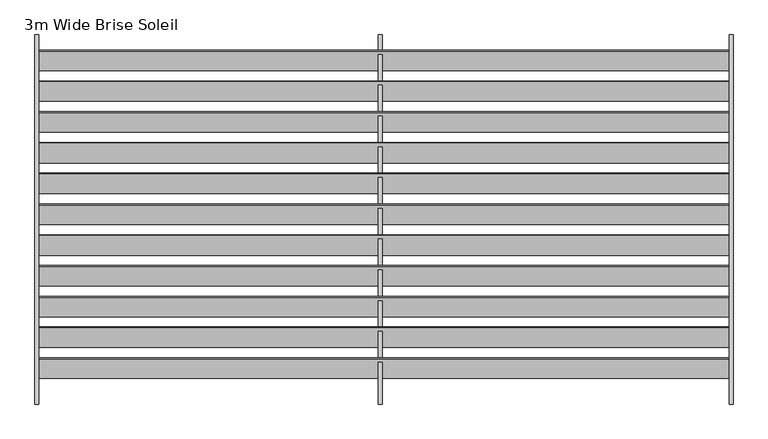
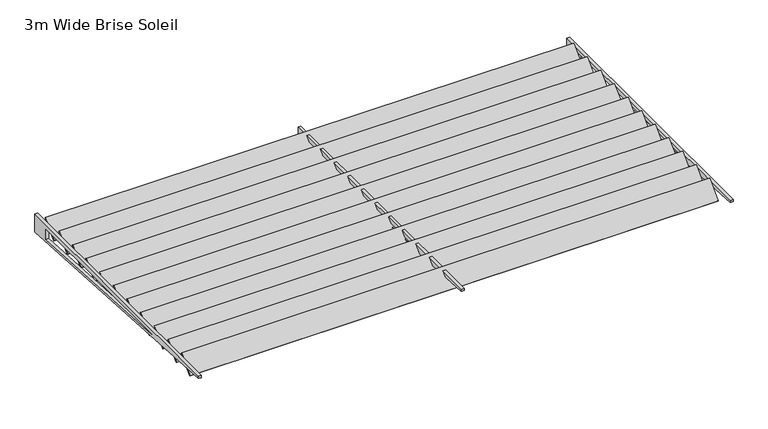
"""IFC4 building model written with IfcOpenShell, lengths in millimetres: railing geometry, 3m Wide Brise Soleil."""

from ifc_helpers import new_model, si_unit, frame, origin, place, context, project, spatial, polyline, outline, extrude, source, transform, mapped, element, save


def railing_3m_wide_brise_soleil_33fbfd34(model_context):
    return source(origin(), model_context, "Body", "SweptSolid", [
        extrude(outline(polyline([(0.0, -10.0), (0.0, 0.0), (5596.1382149, 0.0), (5596.1382149, -10.0), (0.0, -10.0)])), frame((4426.8341559, -31953.9338219, -139.965894), z_axis=(0.0, 0.7071067811931987, 0.7071067811798963), x_axis=(1.0, 0.0, 0.0)), (0.0, 0.0, 1.0), 225.0),
        extrude(outline(polyline([(0.0, -10.0), (0.0, 0.0), (5596.1382149, 0.0), (5596.1382149, -10.0), (0.0, -10.0)])), frame((4426.8341559, -31703.9338219, -139.965894), z_axis=(0.0, 0.7071067811931987, 0.7071067811798963), x_axis=(1.0, 0.0, 0.0)), (0.0, 0.0, 1.0), 225.0),
        extrude(outline(polyline([(0.0, -10.0), (0.0, 0.0), (5596.1382149, 0.0), (5596.1382149, -10.0), (0.0, -10.0)])), frame((4426.8341559, -31453.9338219, -139.965894), z_axis=(0.0, 0.7071067811931987, 0.7071067811798963), x_axis=(1.0, 0.0, 0.0)), (0.0, 0.0, 1.0), 225.0),
        extrude(outline(polyline([(0.0, -10.0), (0.0, 0.0), (5596.1382149, 0.0), (5596.1382149, -10.0), (0.0, -10.0)])), frame((4426.8341559, -31203.9338219, -139.965894), z_axis=(0.0, 0.7071067811931987, 0.7071067811798963), x_axis=(1.0, 0.0, 0.0)), (0.0, 0.0, 1.0), 225.0),
        extrude(outline(polyline([(0.0, -10.0), (0.0, 0.0), (5596.1382149, 0.0), (5596.1382149, -10.0), (0.0, -10.0)])), frame((4426.8341559, -30953.9338219, -139.965894), z_axis=(0.0, 0.7071067811931987, 0.7071067811798963), x_axis=(1.0, 0.0, 0.0)), (0.0, 0.0, 1.0), 225.0),
        extrude(outline(polyline([(0.0, -10.0), (0.0, 0.0), (5596.1382149, 0.0), (5596.1382149, -10.0), (0.0, -10.0)])), frame((4426.8341559, -30703.9338219, -139.965894), z_axis=(0.0, 0.7071067811931987, 0.7071067811798963), x_axis=(1.0, 0.0, 0.0)), (0.0, 0.0, 1.0), 225.0),
        extrude(outline(polyline([(0.0, -10.0), (0.0, 0.0), (5596.1382149, 0.0), (5596.1382149, -10.0), (0.0, -10.0)])), frame((4426.8341559, -30453.9338219, -139.965894), z_axis=(0.0, 0.7071067811931987, 0.7071067811798963), x_axis=(1.0, 0.0, 0.0)), (0.0, 0.0, 1.0), 225.0),
        extrude(outline(polyline([(0.0, -10.0), (0.0, 0.0), (5596.1382149, 0.0), (5596.1382149, -10.0), (0.0, -10.0)])), frame((4426.8341559, -30203.9338219, -139.965894), z_axis=(0.0, 0.7071067811931987, 0.7071067811798963), x_axis=(1.0, 0.0, 0.0)), (0.0, 0.0, 1.0), 225.0),
        extrude(outline(polyline([(0.0, -10.0), (0.0, 0.0), (5596.1382149, 0.0), (5596.1382149, -10.0), (0.0, -10.0)])), frame((4426.8341559, -29953.9338219, -139.965894), z_axis=(0.0, 0.7071067811931987, 0.7071067811798963), x_axis=(1.0, 0.0, 0.0)), (0.0, 0.0, 1.0), 225.0),
        extrude(outline(polyline([(0.0, -10.0), (0.0, 0.0), (5596.1382149, 0.0), (5596.1382149, -10.0), (0.0, -10.0)])), frame((4426.8341559, -29703.9338219, -139.965894), z_axis=(0.0, 0.7071067811931987, 0.7071067811798963), x_axis=(1.0, 0.0, 0.0)), (0.0, 0.0, 1.0), 225.0),
        extrude(outline(polyline([(0.0, -10.0), (0.0, 0.0), (5596.1382149, 0.0), (5596.1382149, -10.0), (0.0, -10.0)])), frame((4426.8341559, -29453.9338219, -139.965894), z_axis=(0.0, 0.7071067811931987, 0.7071067811798963), x_axis=(1.0, 0.0, 0.0)), (0.0, 0.0, 1.0), 225.0),
        extrude(outline(polyline([(-32170.7240302, 0.0), (-29170.7240302, 0.0), (-29170.7240302, -200.0), (-32170.7240302, -25.0), (-32170.7240302, 0.0)]), holes=[polyline([(-29370.7240302, -163.2908347), (-29370.7240302, -50.0), (-31312.8526257, -50.0), (-29370.7240302, -163.2908347)])]), frame((7179.0414006, 0.0, 0.0), z_axis=(1.0, 0.0, 0.0), x_axis=(0.0, 1.0, 0.0)), (0.0, 0.0, 1.0), 30.0),
        extrude(outline(polyline([(-32170.7240302, 0.0), (-29170.7240302, 0.0), (-29170.7240302, -200.0), (-32170.7240302, -25.0), (-32170.7240302, 0.0)]), holes=[polyline([(-29370.7240302, -163.2908347), (-29370.7240302, -50.0), (-31312.8526257, -50.0), (-29370.7240302, -163.2908347)])]), frame((10027.110508, 0.0, 0.0), z_axis=(1.0, 0.0, 0.0), x_axis=(0.0, 1.0, 0.0)), (0.0, 0.0, 1.0), 30.0),
        extrude(outline(polyline([(-32170.7240302, 0.0), (-29170.7240302, 0.0), (-29170.7240302, -200.0), (-32170.7240302, -25.0), (-32170.7240302, 0.0)]), holes=[polyline([(-29370.7240302, -163.2908347), (-29370.7240302, -50.0), (-31312.8526257, -50.0), (-29370.7240302, -163.2908347)])]), frame((4390.9722932, 0.0, 0.0), z_axis=(1.0, 0.0, 0.0), x_axis=(0.0, 1.0, 0.0)), (0.0, 0.0, 1.0), 30.0),
    ])


if __name__ == "__main__":
    model = new_model("IFC4")
    model_context = context("Model", 3, world=origin())
    ifc_project = project(units=[si_unit("LENGTHUNIT", "METRE", prefix="MILLI")], contexts=[model_context])
    site = spatial("IfcSite", under=ifc_project)
    building = spatial("IfcBuilding", under=site)
    placement = place(None, origin())
    railing_3m_wide_brise_soleil_shape = railing_3m_wide_brise_soleil_33fbfd34(model_context)
    element("IfcRailing", 1, ObjectType="3m Wide Brise Soleil", at=placement, inside=building, context=model_context, shape_type="MappedRepresentation", body=[
        mapped(railing_3m_wide_brise_soleil_shape, transform((0.0, 0.0, 0.0), x_axis=(1.0, 0.0, 0.0), y_axis=(0.0, 1.0, 0.0), z_axis=(0.0, 0.0, 1.0))),
    ])
    save(model, "model.ifc")

# Revit data of these elements
# Element 1 (IfcRailing, "3m Wide Brise Soleil")
#   Materials on its faces: "Metal - Aluminium", "Metal - Steel"
# Materials
#   "Metal - Aluminium": class "Unassigned", colour RGB 247 247 247, transparency 0
#   "Metal - Steel": class "Unassigned", colour RGB 199 199 199, transparency 0
